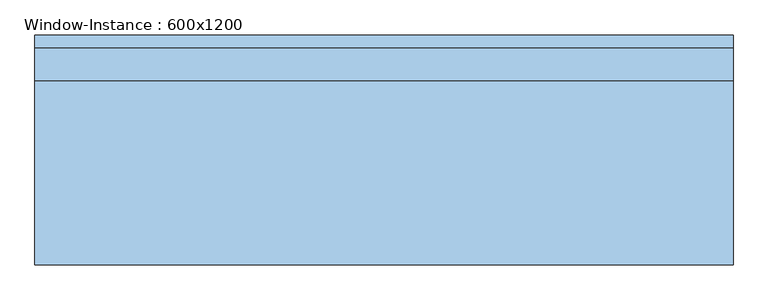
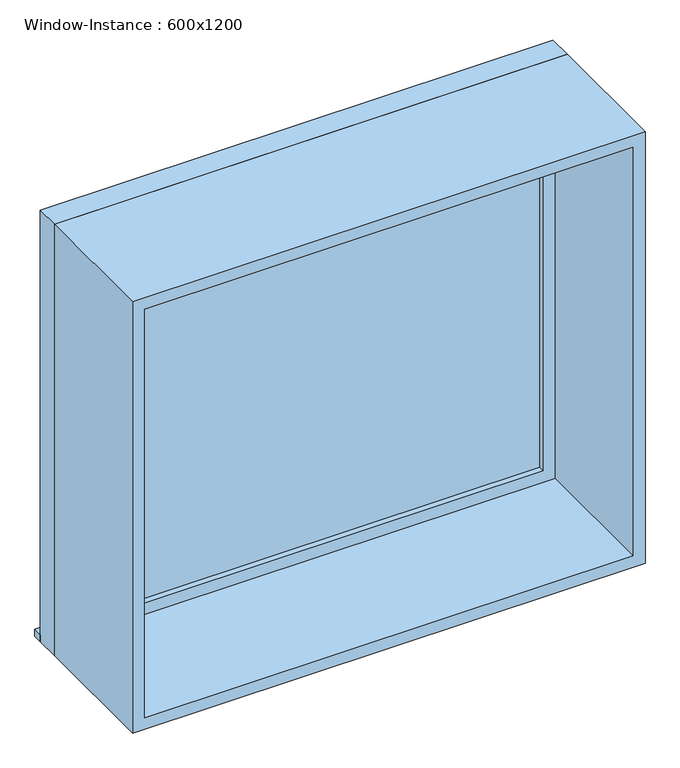
"""IFC4 building model written with IfcOpenShell, lengths in millimetres: window geometry, Window-Instance : 600x1200."""

from ifc_helpers import new_model, si_unit, frame, origin, place, context, project, spatial, polyline, outline, extrude, source, transform, mapped, element, save


def window_instance_600x1200_39196e72(model_context):
    return source(origin(), model_context, "Body", "SweptSolid", [
        extrude(outline(polyline([(-713.1, 235.4), (636.9, 235.4), (636.9, 210.0), (-713.1, 210.0), (-713.1, 235.4)])), frame((0.0, 0.0, 900.0), z_axis=(0.0, 0.0, 1.0), x_axis=(1.0, 0.0, 0.0)), (0.0, 0.0, 1.0), 19.05),
        extrude(outline(polyline([(573.4, 161.425), (-649.6, 161.425), (-649.6, 174.125), (573.4, 174.125), (573.4, 161.425)])), frame((0.0, 0.0, 963.5), z_axis=(0.0, 0.0, 1.0), x_axis=(1.0, 0.0, 0.0)), (0.0, 0.0, 1.0), 1073.0),
        extrude(outline(polyline([(2080.95, -694.05), (919.05, -694.05), (919.05, 617.85), (2080.95, 617.85), (2080.95, -694.05)]), holes=[polyline([(2036.5, -649.6), (2036.5, 573.4), (963.5, 573.4), (963.5, -649.6), (2036.5, -649.6)])]), frame((0.0, 145.55, 0.0), z_axis=(0.0, 1.0, 0.0), x_axis=(0.0, 0.0, 1.0)), (0.0, 0.0, 1.0), 44.45),
        extrude(outline(polyline([(2100.0, -713.1), (900.0, -713.1), (900.0, 636.9), (2100.0, 636.9), (2100.0, -713.1)]), holes=[polyline([(2068.25, -681.35), (2068.25, 605.15), (931.75, 605.15), (931.75, -681.35), (2068.25, -681.35)])]), frame((0.0, -210.0, 0.0), z_axis=(0.0, 1.0, 0.0), x_axis=(0.0, 0.0, 1.0)), (0.0, 0.0, 1.0), 355.55),
        extrude(outline(polyline([(2100.0, 636.9), (2100.0, -713.1), (900.0, -713.1), (900.0, 636.9), (2100.0, 636.9)]), holes=[polyline([(2080.95, 617.85), (919.05, 617.85), (919.05, -694.05), (2080.95, -694.05), (2080.95, 617.85)])]), frame((0.0, 145.55, 0.0), z_axis=(0.0, 1.0, 0.0), x_axis=(0.0, 0.0, 1.0)), (0.0, 0.0, 1.0), 64.45),
    ])


if __name__ == "__main__":
    model = new_model("IFC4")
    model_context = context("Model", 3, world=origin())
    ifc_project = project(units=[si_unit("LENGTHUNIT", "METRE", prefix="MILLI")], contexts=[model_context])
    site = spatial("IfcSite", under=ifc_project)
    building = spatial("IfcBuilding", under=site)
    placement = place(None, origin())
    window_instance_600x1200_shape = window_instance_600x1200_39196e72(model_context)
    element("IfcWindow", 1, ObjectType="Window-Instance : 600x1200", at=placement, inside=building, context=model_context, shape_type="MappedRepresentation", body=[
        mapped(window_instance_600x1200_shape, transform((0.0, 0.0, 0.0), x_axis=(1.0, 0.0, 0.0), y_axis=(0.0, 1.0, 0.0), z_axis=(0.0, 0.0, 1.0))),
    ])
    save(model, "model.ifc")

# Revit data of these elements
# Type "Window-Instance : 600x1200"
#   Type Mark = "7"
#   Construction Type Id = "GSP4R"
#   Assembly Code = "B2020100"
#   Analytic Construction = "1/8 in Pilkington single glazing"
#   Visual Light Transmittance = 0.9
#   Thermal Resistance (R) = 0.149095 (m²·K)/W
#   Solar Heat Gain Coefficient = 0.86
#   Heat Transfer Coefficient (U) = 6.70716 W/(m²·K)
#   Height [instance default] = 1200 mm
#   Default Sill Height = 900 mm
#   Width [instance default] = 600 mm
#   Window Inset = 20 mm
#   Glass Pane Material = WW-EC-GL-Storefront
#   Sash Material = WW-EC-RGB-White
#   Wall Closure = (empty or 0)
# Element 1 (IfcWindow, "Window-Instance : 600x1200")
#   Width = 1350 mm
#   Materials on its faces: "WW-EC-RGB-White", "WW-EC-GL-Storefront"
# Materials
#   "WW-EC-GL-Storefront": class "Glass", colour RGB 236 240 239, transparency 0.85, Description = "Storefront Glass", Cost = 0
#   "WW-EC-RGB-White": class "Generic", colour RGB 255 255 255, transparency 0, Comments = "If region requests off-white, swith asset color to RGB 231-228-220", Description = "Generic Color", Cost = 0
